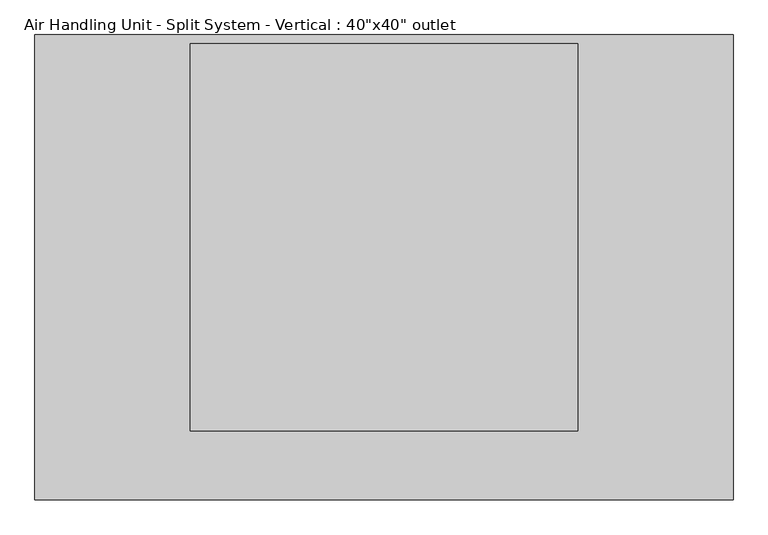
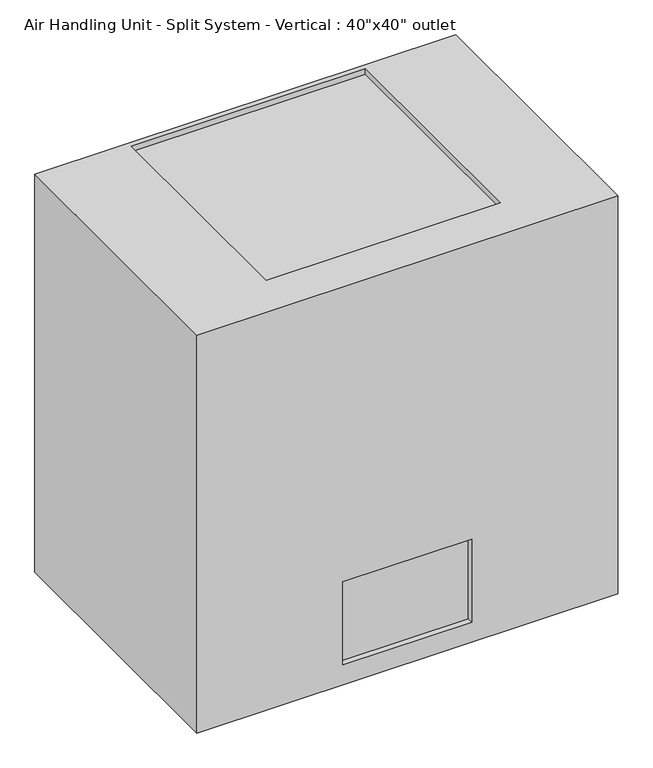
"""IFC4 building model written with IfcOpenShell, lengths in millimetres: proxy geometry."""

import ifcopenshell
import ifcopenshell.guid

model = None  # the IFC model being written
_history = None  # IfcOwnerHistory: only IFC2X3 demands one
_inside = {}  # id of a spatial element -> (the spatial element, [elements in it])
_under = {}  # id of a project, library or spatial element -> (it, [spatial elements below it])
_declared = {}  # id of a project -> (the project, [libraries it declares])
_typed = {}  # id of a type object -> (the type object, [elements of that type])
_made_of = {}  # id of a material, layer set ... -> (it, [elements and type objects made of it])


def new_model(schema):
    """Start an empty IFC model of exactly this schema.

    Asked for "IFC4X3", IfcOpenShell would pick the latest addendum, in which some entities
    have other attributes; the version numbers below select the first issue.
    IFC2X3 requires an IfcOwnerHistory on every rooted entity: one is made here for all.
    """
    global model, _history
    if schema == "IFC4X3":
        model = ifcopenshell.file(schema_version=(4, 3, 0, 0))
    else:
        model = ifcopenshell.file(schema=schema)
    _inside.clear()
    _under.clear()
    _declared.clear()
    _typed.clear()
    _made_of.clear()
    _history = None
    if model.schema == "IFC2X3":
        org = make("IfcOrganization", Name="unknown")
        user = make(
            "IfcPersonAndOrganization",
            ThePerson=make("IfcPerson", FamilyName="unknown"),
            TheOrganization=org,
        )
        app = make(
            "IfcApplication",
            ApplicationDeveloper=org,
            Version="unknown",
            ApplicationFullName="unknown",
            ApplicationIdentifier="unknown",
        )
        _history = make(
            "IfcOwnerHistory",
            OwningUser=user,
            OwningApplication=app,
            ChangeAction="ADDED",
            CreationDate=0,
        )
    return model


def make(cls, **values):
    """One entity of the class cls with the attributes given. An attribute that is None is left unset."""
    return model.create_entity(
        cls, **{name: value for name, value in values.items() if value is not None}
    )


def rooted(cls, **values):
    """An entity with a GlobalId (a new one), such as an element, a storey or a relation."""
    return make(cls, GlobalId=ifcopenshell.guid.new(), OwnerHistory=_history, **values)


def si_unit(unit_type, name, prefix=None):
    """IfcSIUnit, for example si_unit("LENGTHUNIT", "METRE", prefix="MILLI")."""
    return make("IfcSIUnit", UnitType=unit_type, Prefix=prefix, Name=name)


def assignment(units):
    """IfcUnitAssignment: the units of a project."""
    return None if units is None else make("IfcUnitAssignment", Units=units)


def point(xyz):
    """IfcCartesianPoint."""
    return None if xyz is None else make("IfcCartesianPoint", Coordinates=xyz)


def direction(xyz):
    """IfcDirection."""
    return None if xyz is None else make("IfcDirection", DirectionRatios=xyz)


def frame(location, z_axis=None, x_axis=None):
    """IfcAxis2Placement3D, a coordinate frame: its origin and axes. An axis left out is left unset."""
    return make(
        "IfcAxis2Placement3D",
        Location=point(location),
        Axis=direction(z_axis),
        RefDirection=direction(x_axis),
    )


def frame_2d(location, x_axis=None):
    """IfcAxis2Placement2D, a coordinate frame in the plane: its origin and x axis."""
    return make(
        "IfcAxis2Placement2D", Location=point(location), RefDirection=direction(x_axis)
    )


def origin():
    """The frame at (0, 0, 0) with its axes left unset."""
    return frame((0.0, 0.0, 0.0))


def place(relative_to, where):
    """IfcLocalPlacement: puts the frame where relative to a parent placement (None: the world)."""
    return make(
        "IfcLocalPlacement", PlacementRelTo=relative_to, RelativePlacement=where
    )


def context(
    kind, dimensions, precision=None, world=None, true_north=None, identifier=None
):
    """IfcGeometricRepresentationContext, for example the 3D "Model" context."""
    return make(
        "IfcGeometricRepresentationContext",
        ContextIdentifier=identifier,
        ContextType=kind,
        CoordinateSpaceDimension=dimensions,
        Precision=precision,
        WorldCoordinateSystem=world,
        TrueNorth=true_north,
    )


def project(units=None, contexts=None):
    """IfcProject with its units and contexts."""
    return rooted(
        "IfcProject",
        Name="project",
        RepresentationContexts=contexts,
        UnitsInContext=assignment(units),
    )


def spatial(cls, under=None, at=None, **own):
    """A site, building, storey or space (cls), placed at a placement, below another one or the project."""
    s = rooted(cls, ObjectPlacement=at, **own)
    if under is not None:
        _under.setdefault(under.id(), (under, []))[1].append(s)
    return s


def circle_curve(where, radius):
    """IfcCircle in the frame where."""
    return make("IfcCircle", Position=where, Radius=radius)


def trimmed(basis, trim1, trim2, sense, master):
    """IfcTrimmedCurve: the piece of a basis curve between two trims."""
    return make(
        "IfcTrimmedCurve",
        BasisCurve=basis,
        Trim1=trim1,
        Trim2=trim2,
        SenseAgreement=sense,
        MasterRepresentation=master,
    )


def segment(curve, same_sense, transition):
    """IfcCompositeCurveSegment."""
    return make(
        "IfcCompositeCurveSegment",
        Transition=transition,
        SameSense=same_sense,
        ParentCurve=curve,
    )


def composite_curve(segments, self_intersect=None):
    """IfcCompositeCurve: segments joined end to end."""
    return make("IfcCompositeCurve", Segments=segments, SelfIntersect=self_intersect)


def outline(outer, holes=None, kind="AREA"):
    """IfcArbitraryClosedProfileDef: a profile drawn as a closed curve; with holes, ...WithVoids."""
    if holes is None:
        return make("IfcArbitraryClosedProfileDef", ProfileType=kind, OuterCurve=outer)
    return make(
        "IfcArbitraryProfileDefWithVoids",
        ProfileType=kind,
        OuterCurve=outer,
        InnerCurves=holes,
    )


def extrude(swept, where, along, depth):
    """IfcExtrudedAreaSolid: the profile swept, set in the frame where, extruded along a direction by depth."""
    return make(
        "IfcExtrudedAreaSolid",
        SweptArea=swept,
        Position=where,
        ExtrudedDirection=direction(along),
        Depth=depth,
    )


def faces_of(points, faces, orient=None, outer=None):
    """IfcFace entities. A face is a list of loops; a loop is a list of indices into points, from 0.

    orient and outer hold one flag for each loop. By default every Orientation is true, the
    first loop of a face is its IfcFaceOuterBound and the others are IfcFaceBound.
    """
    made = []
    for i, loops in enumerate(faces):
        bounds = []
        for j, loop in enumerate(loops):
            is_outer = j == 0 if outer is None else outer[i][j]
            bounds.append(
                make(
                    "IfcFaceOuterBound" if is_outer else "IfcFaceBound",
                    Bound=make("IfcPolyLoop", Polygon=[points[k] for k in loop]),
                    Orientation=True if orient is None else orient[i][j],
                )
            )
        made.append(make("IfcFace", Bounds=bounds))
    return made


def faceted_brep(points, faces, orient=None, outer=None, voids=None):
    """IfcFacetedBrep: a solid bounded by flat faces; with voids (closed shells), ...WithVoids."""
    shared = [point(p) for p in points]
    hull = make("IfcClosedShell", CfsFaces=faces_of(shared, faces, orient, outer))
    if voids is None:
        return make("IfcFacetedBrep", Outer=hull)
    return make(
        "IfcFacetedBrepWithVoids",
        Outer=hull,
        Voids=[
            make(cls, CfsFaces=faces_of(shared, fs, o, b)) for cls, fs, o, b in voids
        ],
    )


def shape(context_of_items, identifier, shape_type, items):
    """IfcShapeRepresentation: the items that make up one representation, for example the "Body"."""
    return make(
        "IfcShapeRepresentation",
        ContextOfItems=context_of_items,
        RepresentationIdentifier=identifier,
        RepresentationType=shape_type,
        Items=items,
    )


def source(mapping_origin, context_of_items, identifier, shape_type, items):
    """IfcRepresentationMap: a shape defined once, which mapped items show again and again."""
    return make(
        "IfcRepresentationMap",
        MappingOrigin=mapping_origin,
        MappedRepresentation=shape(context_of_items, identifier, shape_type, items),
    )


def transform(
    local_origin,
    x_axis=None,
    y_axis=None,
    z_axis=None,
    scale=None,
    scale2=None,
    scale3=None,
    uniform=True,
):
    """IfcCartesianTransformationOperator3D, or its non-uniform kind. x_axis, y_axis, z_axis: its Axis1, 2, 3."""
    if uniform:
        return make(
            "IfcCartesianTransformationOperator3D",
            Axis1=direction(x_axis),
            Axis2=direction(y_axis),
            LocalOrigin=point(local_origin),
            Scale=scale,
            Axis3=direction(z_axis),
        )
    return make(
        "IfcCartesianTransformationOperator3DnonUniform",
        Axis1=direction(x_axis),
        Axis2=direction(y_axis),
        LocalOrigin=point(local_origin),
        Scale=scale,
        Axis3=direction(z_axis),
        Scale2=scale2,
        Scale3=scale3,
    )


def mapped(mapping_source, mapping_target):
    """IfcMappedItem: shows the shape of a source again, moved by a transform."""
    return make(
        "IfcMappedItem", MappingSource=mapping_source, MappingTarget=mapping_target
    )


def made_of(thing, what):
    """Note that an element or type object is made of a material, layer set ...; save() writes the relation."""
    if what is not None:
        _made_of.setdefault(what.id(), (what, []))[1].append(thing)
    return thing


def element(
    cls,
    number,
    at=None,
    inside=None,
    cuts=None,
    type_object=None,
    material=None,
    context=None,
    identifier="Body",
    shape_type=None,
    held_by="IfcProductDefinitionShape",
    body=None,
    shapes=None,
    **own,
):
    """One element of the class cls, such as IfcWall. Its Tag is "e" and its number.

    at: its placement. inside: the storey or other place that contains it. cuts: it is an
    opening in that element (IfcRelVoidsElement). A single representation is given by context,
    identifier, shape_type and body (its items); several are given by shapes. held_by: the class
    of the entity that holds the representations. save() writes the other relations.
    """
    e = rooted(cls, Tag="e%d" % number, ObjectPlacement=at, **own)
    if body is not None:
        shapes = [shape(context, identifier, shape_type, body)]
    if shapes is not None:
        e.Representation = make(held_by, Representations=shapes)
    if inside is not None:
        _inside.setdefault(inside.id(), (inside, []))[1].append(e)
    if cuts is not None:
        rooted(
            "IfcRelVoidsElement", RelatingBuildingElement=cuts, RelatedOpeningElement=e
        )
    if type_object is not None:
        _typed.setdefault(type_object.id(), (type_object, []))[1].append(e)
    return made_of(e, material)


def aggregate(whole, parts):
    """IfcRelAggregates: a whole, such as a stair, and the parts it consists of."""
    return rooted("IfcRelAggregates", RelatingObject=whole, RelatedObjects=parts)


def save(model, path):
    """Write the relations noted so far, then the file.

    IfcRelAggregates (storeys below a building ...), IfcRelContainedInSpatialStructure (elements
    in a storey), IfcRelDefinesByType, IfcRelAssociatesMaterial and IfcRelDeclares: one each for
    every whole, place, type object, material and project.
    """
    for whole, parts in _under.values():
        aggregate(whole, parts)
    for where, things in _inside.values():
        rooted(
            "IfcRelContainedInSpatialStructure",
            RelatedElements=things,
            RelatingStructure=where,
        )
    for kind, things in _typed.values():
        rooted("IfcRelDefinesByType", RelatedObjects=things, RelatingType=kind)
    for what, things in _made_of.values():
        rooted("IfcRelAssociatesMaterial", RelatedObjects=things, RelatingMaterial=what)
    for by, libraries in _declared.values():
        rooted("IfcRelDeclares", RelatingContext=by, RelatedDefinitions=libraries)
    model.write(path)


def proxy_8db298f6(model_context):
    return source(origin(), model_context, "Body", "SolidModel", [
        extrude(outline(composite_curve([segment(trimmed(circle_curve(frame_2d((132.55625, -866.378125)), 9.525), [point((142.08125, -866.378125))], [point((123.03125, -866.378125))], False, "CARTESIAN"), True, "CONTINUOUS"), segment(trimmed(circle_curve(frame_2d((132.55625, -866.378125)), 9.525), [point((123.03125, -866.378125))], [point((142.08125, -866.378125))], False, "CARTESIAN"), True, "CONTINUOUS")], self_intersect=False)), frame((0.0, 287.0398438, 0.0), z_axis=(0.0, 1.0, 0.0), x_axis=(0.0, 0.0, 1.0)), (0.0, 0.0, 1.0), 25.4),
        extrude(outline(composite_curve([segment(trimmed(circle_curve(frame_2d((394.096875, 815.975)), 4.7625), [point((398.859375, 815.975))], [point((389.334375, 815.975))], False, "CARTESIAN"), True, "CONTINUOUS"), segment(trimmed(circle_curve(frame_2d((394.096875, 815.975)), 4.7625), [point((389.334375, 815.975))], [point((398.859375, 815.975))], False, "CARTESIAN"), True, "CONTINUOUS")], self_intersect=False)), frame((0.0, 287.0398438, 0.0), z_axis=(0.0, 1.0, 0.0), x_axis=(0.0, 0.0, 1.0)), (0.0, 0.0, 1.0), 25.4),
        extrude(outline(composite_curve([segment(trimmed(circle_curve(frame_2d((465.534375, 815.975)), 14.2875), [point((479.821875, 815.975))], [point((451.246875, 815.975))], False, "CARTESIAN"), True, "CONTINUOUS"), segment(trimmed(circle_curve(frame_2d((465.534375, 815.975)), 14.2875), [point((451.246875, 815.975))], [point((479.821875, 815.975))], False, "CARTESIAN"), True, "CONTINUOUS")], self_intersect=False)), frame((0.0, 287.0398438, 0.0), z_axis=(0.0, 1.0, 0.0), x_axis=(0.0, 0.0, 1.0)), (0.0, 0.0, 1.0), 25.4),
        faceted_brep([(914.4, 609.6, 1828.8), (-914.4, 609.6, 1828.8), (-914.4, -609.6, 1828.8), (914.4, -609.6, 1828.8), (508.0, 586.7796875, 1828.8), (508.0, -429.2203125, 1828.8), (-508.0, -429.2203125, 1828.8), (-508.0, 586.7796875, 1828.8), (914.4, 609.6, 0.0), (914.4, -609.6, 0.0), (-914.4, -609.6, 0.0), (-914.4, 609.6, 0.0), (279.4, -609.6, 472.8765625), (279.4, -609.6, 91.8765625), (-279.4, -609.6, 91.8765625), (-279.4, -609.6, 472.8765625), (508.0, 586.7796875, 1803.4), (-508.0, 586.7796875, 1803.4), (-508.0, -429.2203125, 1803.4), (508.0, -429.2203125, 1803.4), (279.4, -584.2, 472.8765625), (-279.4, -584.2, 472.8765625), (-279.4, -584.2, 91.8765625), (279.4, -584.2, 91.8765625)], [[[0, 1, 2, 3], [4, 5, 6, 7]], [[8, 9, 10, 11]], [[1, 0, 8, 11]], [[2, 1, 11, 10]], [[3, 2, 10, 9], [12, 13, 14, 15]], [[0, 3, 9, 8]], [[16, 17, 18, 19]], [[16, 19, 5, 4]], [[19, 18, 6, 5]], [[18, 17, 7, 6]], [[17, 16, 4, 7]], [[20, 21, 22, 23]], [[20, 23, 13, 12]], [[23, 22, 14, 13]], [[22, 21, 15, 14]], [[21, 20, 12, 15]]]),
    ])


if __name__ == "__main__":
    model = new_model("IFC4")
    model_context = context("Model", 3, world=origin())
    ifc_project = project(units=[si_unit("LENGTHUNIT", "METRE", prefix="MILLI")], contexts=[model_context])
    site = spatial("IfcSite", under=ifc_project)
    building = spatial("IfcBuilding", under=site)
    placement = place(None, origin())
    proxy_shape = proxy_8db298f6(model_context)
    element("IfcBuildingElementProxy", 1, Name="Air Handling Unit - Split System - Vertical : 40\"x40\" outlet", ObjectType="Air Handling Unit - Split System - Vertical : 40\"x40\" outlet", at=placement, inside=building, context=model_context, shape_type="MappedRepresentation", body=[
        mapped(proxy_shape, transform((0.0, 0.0, 0.0), x_axis=(1.0, 0.0, 0.0), y_axis=(0.0, 1.0, 0.0), z_axis=(0.0, 0.0, 1.0))),
    ])
    save(model, "model.ifc")

# Revit data of these elements
# Project information
#   Project Issue Date = "Issue Date"
#   Project Status = "Project Status"
#   Client Name = "Owner"
#   Project Address = "Enter address here"
#   Project Name = "Project Name"
#   Project Number = "Project Number"
# Type "Air Handling Unit - Split System - Vertical : 40\"x40\" outlet"
#   PartShape = "Rectangular Duct"
#   Model = "03"
#   Voltage = 208 V
#   UnitWidth = 6' - 0"
#   UnitHeight = 6' - 0"
#   UnitDepth = 4' - 0"
#   Width1 = 3' - 4"
#   SupplyOpeningOffset = 0' - 0 115/128"
#   Outlet Radius = 9/16"
#   Outlet Diameter = 1 1/8"
#   Inlet Radius = 3/16"
#   Inlet Diameter = 3/8"
#   Height1 = 3' - 4"
#   SupplyConnectorOffset = 1' - 8"
#   Width2 = 1' - 10"
#   Height2 = 1' - 3"
#   ReturnConnectorOffset = 0' - 7 1/2"
#   ReturnAirOffset = 0' - 3 79/128"
#   Half UnitWidth = 3' - 0"
#   Drain Flow [instance default] = 0 GPM
#   C3 Offset 1 = 1' - 6 21/64"
#   Apparent Load = 10816 VA
#   External Static Pressure [instance default] = 0.50 in-wg
#   Air Flow [instance default] = 1170 CFM
#   Number of Poles = 3
#   Load Classification = Cooling
#   Assembly Code = ""
